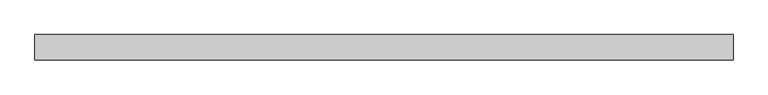
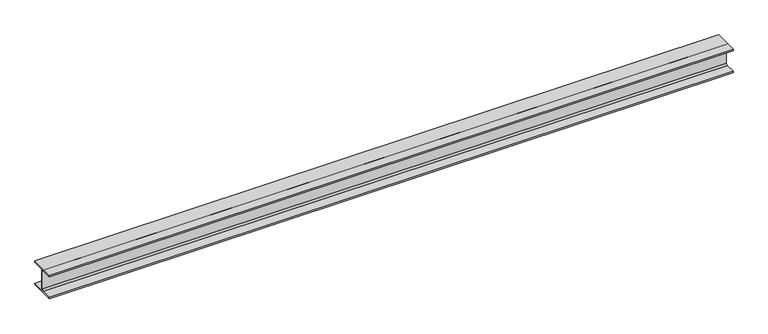
"""IFC4 building model written with IfcOpenShell, lengths in millimetres: beam geometry, 0912_Steel Framing_H-KSD3502 : H_SB_ASB_H-200x200x8x12."""

import ifcopenshell
import ifcopenshell.guid

model = None  # the IFC model being written
_history = None  # IfcOwnerHistory: only IFC2X3 demands one
_inside = {}  # id of a spatial element -> (the spatial element, [elements in it])
_under = {}  # id of a project, library or spatial element -> (it, [spatial elements below it])
_declared = {}  # id of a project -> (the project, [libraries it declares])
_typed = {}  # id of a type object -> (the type object, [elements of that type])
_made_of = {}  # id of a material, layer set ... -> (it, [elements and type objects made of it])


def new_model(schema):
    """Start an empty IFC model of exactly this schema.

    Asked for "IFC4X3", IfcOpenShell would pick the latest addendum, in which some entities
    have other attributes; the version numbers below select the first issue.
    IFC2X3 requires an IfcOwnerHistory on every rooted entity: one is made here for all.
    """
    global model, _history
    if schema == "IFC4X3":
        model = ifcopenshell.file(schema_version=(4, 3, 0, 0))
    else:
        model = ifcopenshell.file(schema=schema)
    _inside.clear()
    _under.clear()
    _declared.clear()
    _typed.clear()
    _made_of.clear()
    _history = None
    if model.schema == "IFC2X3":
        org = make("IfcOrganization", Name="unknown")
        user = make(
            "IfcPersonAndOrganization",
            ThePerson=make("IfcPerson", FamilyName="unknown"),
            TheOrganization=org,
        )
        app = make(
            "IfcApplication",
            ApplicationDeveloper=org,
            Version="unknown",
            ApplicationFullName="unknown",
            ApplicationIdentifier="unknown",
        )
        _history = make(
            "IfcOwnerHistory",
            OwningUser=user,
            OwningApplication=app,
            ChangeAction="ADDED",
            CreationDate=0,
        )
    return model


def make(cls, **values):
    """One entity of the class cls with the attributes given. An attribute that is None is left unset."""
    return model.create_entity(
        cls, **{name: value for name, value in values.items() if value is not None}
    )


def rooted(cls, **values):
    """An entity with a GlobalId (a new one), such as an element, a storey or a relation."""
    return make(cls, GlobalId=ifcopenshell.guid.new(), OwnerHistory=_history, **values)


def si_unit(unit_type, name, prefix=None):
    """IfcSIUnit, for example si_unit("LENGTHUNIT", "METRE", prefix="MILLI")."""
    return make("IfcSIUnit", UnitType=unit_type, Prefix=prefix, Name=name)


def assignment(units):
    """IfcUnitAssignment: the units of a project."""
    return None if units is None else make("IfcUnitAssignment", Units=units)


def point(xyz):
    """IfcCartesianPoint."""
    return None if xyz is None else make("IfcCartesianPoint", Coordinates=xyz)


def direction(xyz):
    """IfcDirection."""
    return None if xyz is None else make("IfcDirection", DirectionRatios=xyz)


def frame(location, z_axis=None, x_axis=None):
    """IfcAxis2Placement3D, a coordinate frame: its origin and axes. An axis left out is left unset."""
    return make(
        "IfcAxis2Placement3D",
        Location=point(location),
        Axis=direction(z_axis),
        RefDirection=direction(x_axis),
    )


def frame_2d(location, x_axis=None):
    """IfcAxis2Placement2D, a coordinate frame in the plane: its origin and x axis."""
    return make(
        "IfcAxis2Placement2D", Location=point(location), RefDirection=direction(x_axis)
    )


def origin():
    """The frame at (0, 0, 0) with its axes left unset."""
    return frame((0.0, 0.0, 0.0))


def place(relative_to, where):
    """IfcLocalPlacement: puts the frame where relative to a parent placement (None: the world)."""
    return make(
        "IfcLocalPlacement", PlacementRelTo=relative_to, RelativePlacement=where
    )


def context(
    kind, dimensions, precision=None, world=None, true_north=None, identifier=None
):
    """IfcGeometricRepresentationContext, for example the 3D "Model" context."""
    return make(
        "IfcGeometricRepresentationContext",
        ContextIdentifier=identifier,
        ContextType=kind,
        CoordinateSpaceDimension=dimensions,
        Precision=precision,
        WorldCoordinateSystem=world,
        TrueNorth=true_north,
    )


def project(units=None, contexts=None):
    """IfcProject with its units and contexts."""
    return rooted(
        "IfcProject",
        Name="project",
        RepresentationContexts=contexts,
        UnitsInContext=assignment(units),
    )


def spatial(cls, under=None, at=None, **own):
    """A site, building, storey or space (cls), placed at a placement, below another one or the project."""
    s = rooted(cls, ObjectPlacement=at, **own)
    if under is not None:
        _under.setdefault(under.id(), (under, []))[1].append(s)
    return s


def polyline(points):
    """IfcPolyline through the points."""
    return make("IfcPolyline", Points=[point(p) for p in points])


def circle_curve(where, radius):
    """IfcCircle in the frame where."""
    return make("IfcCircle", Position=where, Radius=radius)


def trimmed(basis, trim1, trim2, sense, master):
    """IfcTrimmedCurve: the piece of a basis curve between two trims."""
    return make(
        "IfcTrimmedCurve",
        BasisCurve=basis,
        Trim1=trim1,
        Trim2=trim2,
        SenseAgreement=sense,
        MasterRepresentation=master,
    )


def segment(curve, same_sense, transition):
    """IfcCompositeCurveSegment."""
    return make(
        "IfcCompositeCurveSegment",
        Transition=transition,
        SameSense=same_sense,
        ParentCurve=curve,
    )


def composite_curve(segments, self_intersect=None):
    """IfcCompositeCurve: segments joined end to end."""
    return make("IfcCompositeCurve", Segments=segments, SelfIntersect=self_intersect)


def outline(outer, holes=None, kind="AREA"):
    """IfcArbitraryClosedProfileDef: a profile drawn as a closed curve; with holes, ...WithVoids."""
    if holes is None:
        return make("IfcArbitraryClosedProfileDef", ProfileType=kind, OuterCurve=outer)
    return make(
        "IfcArbitraryProfileDefWithVoids",
        ProfileType=kind,
        OuterCurve=outer,
        InnerCurves=holes,
    )


def extrude(swept, where, along, depth):
    """IfcExtrudedAreaSolid: the profile swept, set in the frame where, extruded along a direction by depth."""
    return make(
        "IfcExtrudedAreaSolid",
        SweptArea=swept,
        Position=where,
        ExtrudedDirection=direction(along),
        Depth=depth,
    )


def shape(context_of_items, identifier, shape_type, items):
    """IfcShapeRepresentation: the items that make up one representation, for example the "Body"."""
    return make(
        "IfcShapeRepresentation",
        ContextOfItems=context_of_items,
        RepresentationIdentifier=identifier,
        RepresentationType=shape_type,
        Items=items,
    )


def source(mapping_origin, context_of_items, identifier, shape_type, items):
    """IfcRepresentationMap: a shape defined once, which mapped items show again and again."""
    return make(
        "IfcRepresentationMap",
        MappingOrigin=mapping_origin,
        MappedRepresentation=shape(context_of_items, identifier, shape_type, items),
    )


def transform(
    local_origin,
    x_axis=None,
    y_axis=None,
    z_axis=None,
    scale=None,
    scale2=None,
    scale3=None,
    uniform=True,
):
    """IfcCartesianTransformationOperator3D, or its non-uniform kind. x_axis, y_axis, z_axis: its Axis1, 2, 3."""
    if uniform:
        return make(
            "IfcCartesianTransformationOperator3D",
            Axis1=direction(x_axis),
            Axis2=direction(y_axis),
            LocalOrigin=point(local_origin),
            Scale=scale,
            Axis3=direction(z_axis),
        )
    return make(
        "IfcCartesianTransformationOperator3DnonUniform",
        Axis1=direction(x_axis),
        Axis2=direction(y_axis),
        LocalOrigin=point(local_origin),
        Scale=scale,
        Axis3=direction(z_axis),
        Scale2=scale2,
        Scale3=scale3,
    )


def mapped(mapping_source, mapping_target):
    """IfcMappedItem: shows the shape of a source again, moved by a transform."""
    return make(
        "IfcMappedItem", MappingSource=mapping_source, MappingTarget=mapping_target
    )


def made_of(thing, what):
    """Note that an element or type object is made of a material, layer set ...; save() writes the relation."""
    if what is not None:
        _made_of.setdefault(what.id(), (what, []))[1].append(thing)
    return thing


def element(
    cls,
    number,
    at=None,
    inside=None,
    cuts=None,
    type_object=None,
    material=None,
    context=None,
    identifier="Body",
    shape_type=None,
    held_by="IfcProductDefinitionShape",
    body=None,
    shapes=None,
    **own,
):
    """One element of the class cls, such as IfcWall. Its Tag is "e" and its number.

    at: its placement. inside: the storey or other place that contains it. cuts: it is an
    opening in that element (IfcRelVoidsElement). A single representation is given by context,
    identifier, shape_type and body (its items); several are given by shapes. held_by: the class
    of the entity that holds the representations. save() writes the other relations.
    """
    e = rooted(cls, Tag="e%d" % number, ObjectPlacement=at, **own)
    if body is not None:
        shapes = [shape(context, identifier, shape_type, body)]
    if shapes is not None:
        e.Representation = make(held_by, Representations=shapes)
    if inside is not None:
        _inside.setdefault(inside.id(), (inside, []))[1].append(e)
    if cuts is not None:
        rooted(
            "IfcRelVoidsElement", RelatingBuildingElement=cuts, RelatedOpeningElement=e
        )
    if type_object is not None:
        _typed.setdefault(type_object.id(), (type_object, []))[1].append(e)
    return made_of(e, material)


def aggregate(whole, parts):
    """IfcRelAggregates: a whole, such as a stair, and the parts it consists of."""
    return rooted("IfcRelAggregates", RelatingObject=whole, RelatedObjects=parts)


def save(model, path):
    """Write the relations noted so far, then the file.

    IfcRelAggregates (storeys below a building ...), IfcRelContainedInSpatialStructure (elements
    in a storey), IfcRelDefinesByType, IfcRelAssociatesMaterial and IfcRelDeclares: one each for
    every whole, place, type object, material and project.
    """
    for whole, parts in _under.values():
        aggregate(whole, parts)
    for where, things in _inside.values():
        rooted(
            "IfcRelContainedInSpatialStructure",
            RelatedElements=things,
            RelatingStructure=where,
        )
    for kind, things in _typed.values():
        rooted("IfcRelDefinesByType", RelatedObjects=things, RelatingType=kind)
    for what, things in _made_of.values():
        rooted("IfcRelAssociatesMaterial", RelatedObjects=things, RelatingMaterial=what)
    for by, libraries in _declared.values():
        rooted("IfcRelDeclares", RelatingContext=by, RelatedDefinitions=libraries)
    model.write(path)


def beam_25d4bc8c(model_context):
    return source(origin(), model_context, "Body", "SweptSolid", [
        extrude(outline(composite_curve([segment(polyline([(100.0, -88.0), (100.0, -100.0), (-100.0, -100.0), (-100.0, -88.0), (-17.0, -88.0)]), True, "CONTINUOUS"), segment(trimmed(circle_curve(frame_2d((-17.0, -75.0)), 13.0), [point((-17.0, -88.0))], [point((-4.0, -75.0))], True, "CARTESIAN"), True, "CONTINUOUS"), segment(polyline([(-4.0, -75.0), (-4.0, 75.0)]), True, "CONTINUOUS"), segment(trimmed(circle_curve(frame_2d((-17.0, 75.0)), 13.0), [point((-4.0, 75.0))], [point((-17.0, 88.0))], True, "CARTESIAN"), True, "CONTINUOUS"), segment(polyline([(-17.0, 88.0), (-100.0, 88.0), (-100.0, 100.0), (100.0, 100.0), (100.0, 88.0), (17.0, 88.0)]), True, "CONTINUOUS"), segment(trimmed(circle_curve(frame_2d((17.0, 75.0)), 13.0), [point((17.0, 88.0))], [point((4.0, 75.0))], True, "CARTESIAN"), True, "CONTINUOUS"), segment(polyline([(4.0, 75.0), (4.0, -75.0)]), True, "CONTINUOUS"), segment(trimmed(circle_curve(frame_2d((17.0, -75.0)), 13.0), [point((4.0, -75.0))], [point((17.0, -88.0))], True, "CARTESIAN"), True, "CONTINUOUS"), segment(polyline([(17.0, -88.0), (100.0, -88.0)]), True, "CONTINUOUS")], self_intersect=False)), frame((-2548.5286375, 0.0, 0.0), z_axis=(1.0, 0.0, 0.0), x_axis=(0.0, 1.0, 0.0)), (0.0, 0.0, 1.0), 5471.23329),
    ])


if __name__ == "__main__":
    model = new_model("IFC4")
    model_context = context("Model", 3, world=origin())
    ifc_project = project(units=[si_unit("LENGTHUNIT", "METRE", prefix="MILLI")], contexts=[model_context])
    site = spatial("IfcSite", under=ifc_project)
    building = spatial("IfcBuilding", under=site)
    placement = place(None, origin())
    beam_shape = beam_25d4bc8c(model_context)
    element("IfcBeam", 1, ObjectType="0912_Steel Framing_H-KSD3502 : H_SB_ASB_H-200x200x8x12", at=placement, inside=building, context=model_context, shape_type="MappedRepresentation", body=[
        mapped(beam_shape, transform((0.0, 0.0, 0.0), x_axis=(1.0, 0.0, 0.0), y_axis=(0.0, 1.0, 0.0), z_axis=(0.0, 0.0, 1.0))),
    ])
    save(model, "model.ifc")

# Revit data of these elements
# Type "0912_Steel Framing_H-KSD3502 : H_SB_ASB_H-200x200x8x12"
#   H_WM Code_1 = "S01AA002-00001 | Main Steel Structure Fabrication Work | Shelter/Building | Medium Steel - Standard (90KG/M>Weight≥30KG/M) | Material: (   )"
#   H_WM Code_2 = "S03AA028-00001 | Main Steel Structure Erection Work | Shelter/Building | Medium Steel (90KG/M>Weight≥30KG/M) | Material: (   )"
#   H_WM Code_3 = "S01AA010-00001 | Main Steel Structure Fabrication Work | Shelter/Building | Steel Painting/Coating | for Non-Fireproofed Steel Surface, Surface Preparation, Primer, Second & Final Coat | Material: (   )"
#   H_Q'ty Cal Type Tag = "SB-Q2"
#   Width = 20.0 cm
#   Web Thickness = 0.8 cm
#   Web Fillet = 1.3 cm
#   Warping Constant = 141000.0 cm⁶
#   W = 0
#   Torsional Moment of Inertia = 26.2485 cm⁴
#   Section Area = 63.53 cm²
#   Plastic Modulus weak axis = 244.0 cm³
#   Plastic Modulus strong axis = 525.0 cm³
#   Perimeter = 1.16 m²/m
#   Nominal Weight = 49.90 kgf/m
#   Moment of Inertia weak axis = 1600.00 cm⁴
#   Moment of Inertia strong axis = 4720.00 cm⁴
#   Height = 20.0 cm
#   Flange Thickness = 1.2 cm
#   Elastic Modulus weak axis = 160.0 cm³
#   Elastic Modulus strong axis = 472.0 cm³
#   Centroid Vertical = 10.0 cm
#   Centroid Horizontal = 10.0 cm
#   Ix = 47200000
#   Length [instance default] = 1.5240 m
#   Zx = 525000
#   b = 0.2000 m
#   h = 0.2000 m
#   r = 0.0130 m
#   s = 0.0080 m
#   t = 0.0120 m
#   A = 0.006353 m²
#   Structural Material [instance default] = Steel, 45-345
#   Assembly Code = ""
# Element 1 (IfcBeam, "0912_Steel Framing_H-KSD3502 : H_SB_ASB_H-200x200x8x12")
#   Structural Material = none
# Materials
#   "Steel, 45-345": class "Metal", colour RGB 189 187 185, transparency 0, Description = "Steel 345 MPa", Cost = 0
